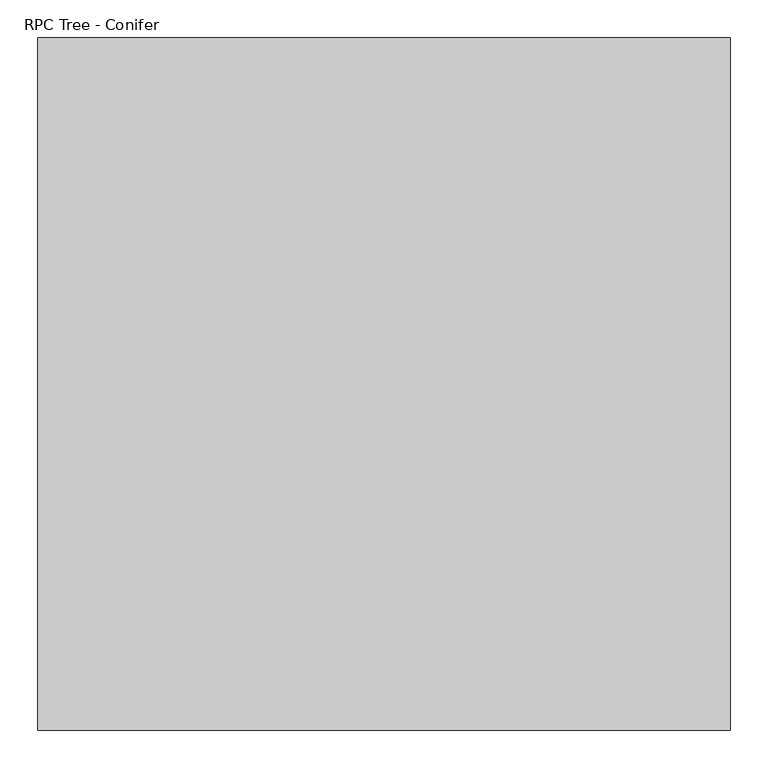
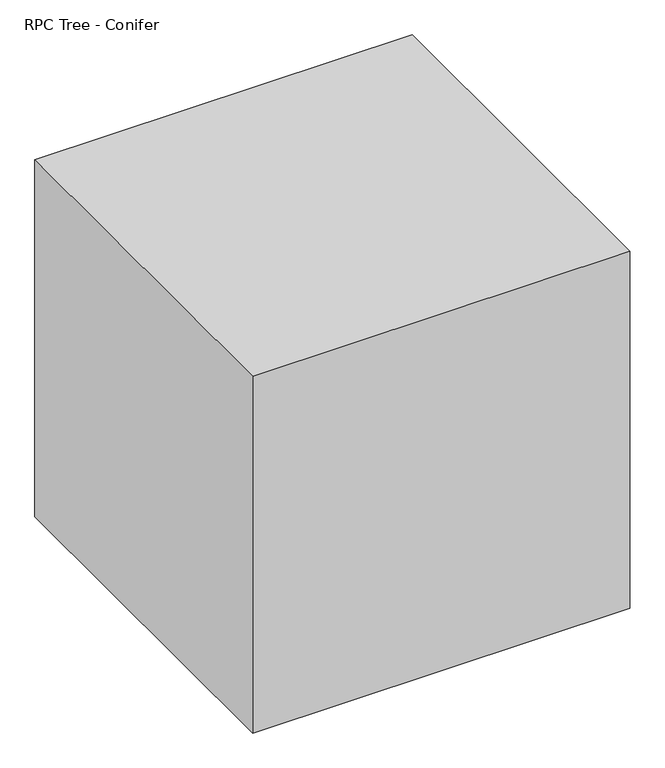
"""IFC4 building model written with IfcOpenShell, lengths in millimetres: geographic element geometry, RPC Tree - Conifer : Colorado Spruce - 4.0 Meters."""

from ifc_helpers import new_model, si_unit, origin, origin_with_axes, place, context, project, spatial, polyline, outline, extrude, source, transform, mapped, element, save


def rpc_tree_conifer_625bb648(model_context):
    return source(origin(), model_context, "Body", "SweptSolid", [
        extrude(outline(polyline([(-457.0033289, -457.2), (-457.0033289, 457.2), (457.3966711, 457.2), (457.3966711, -457.2), (-457.0033289, -457.2)])), origin_with_axes(), (0.0, 0.0, 1.0), 914.4),
    ])


if __name__ == "__main__":
    model = new_model("IFC4")
    model_context = context("Model", 3, world=origin())
    ifc_project = project(units=[si_unit("LENGTHUNIT", "METRE", prefix="MILLI")], contexts=[model_context])
    site = spatial("IfcSite", under=ifc_project)
    building = spatial("IfcBuilding", under=site)
    placement = place(None, origin())
    rpc_tree_conifer_shape = rpc_tree_conifer_625bb648(model_context)
    element("IfcGeographicElement", 1, ObjectType="RPC Tree - Conifer : Colorado Spruce - 4.0 Meters", at=placement, inside=building, context=model_context, shape_type="MappedRepresentation", body=[
        mapped(rpc_tree_conifer_shape, transform((0.0, 0.0, 0.0), x_axis=(1.0, 0.0, 0.0), y_axis=(0.0, 1.0, 0.0), z_axis=(0.0, 0.0, 1.0))),
    ])
    save(model, "model.ifc")

# Revit data of these elements
# Project information
#   Project Status = "Project Status"
#   Client Name = "Revit Project"
#   Project Address = "LIMERICK INSTITUTE of TECHNOLOGY"
#   Project Name = "Commercial Units"
#   Project Number = "01"
# Type "RPC Tree - Conifer : Colorado Spruce - 4.0 Meters"
#   built-in parameter 1005198 = "{2, 15},{39, RPC-16-G0M4-N9PX-U6TN-C000-ST1L-LVER-AU},{1, 0},{1, 0},{2, 13},{1, 8},{5, Color},{1, 0},{1, 0},{3, 0.8},{3, 0.8},{3, 0.8},{1, 8},{7, BBoxMin},{1, 0},{1, 0},{1, 0},{1, 0},{1, 0},{1, 8},{7, BBoxMax},{1, 0},{1, 0},{1, 0},{1, 0},{1, 0},{2, 11},{9, RPCTypeId},{1, 0},{1, 0},{39, RPC-16-G0M4-N9PX-U6TN-C000-ST1L-LVER-AU},{1, 6},{14, RPCPlantHeight},{1, 0},{1, 0},{7, 13.1234},{2, 11},{7, keyword},{1, 0},{1, 0},{34, :RPCs:Trees [General]:Geometry:RPC},{2, 11},{8, category},{1, 0},{1, 0},{15, Trees [General]},{2, 11},{12, LocalizedUID},{1, 0},{1, 0},{15, Colorado Spruce},{2, 14},{6, Height},{1, 0},{1, 0},{7, 13.1234},{1, 2},{16, Cast Reflections},{1, 0},{1, 0},{1, 0},{1, 2},{12, Cast Shadows},{1, 0},{1, 0},{1, 1},{1, 2},{9, Lock View},{1, 0},{1, 0},{1, 0},{1, 4},{5, ViewC},{1, 0},{1, 0},{1, 0},{21, assetlibrary_base.fbx},{1, 5},"
#   built-in parameter 1005195 = "RPC-16-G0M4-N9PX-U6TN-C000-ST1L-LVER-AU"
#   Type Comments = "Colorado Spruce"
#   Height = 4000 mm
#   Description = (empty or 0)
#   Default Elevation = 0
